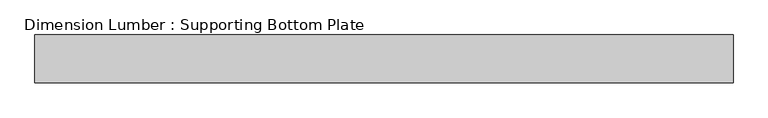
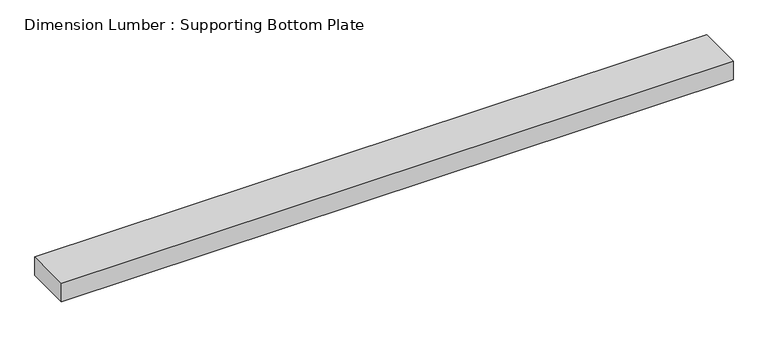
"""IFC4 building model written with IfcOpenShell, lengths in millimetres: beam geometry, Dimension Lumber : Supporting Bottom Plate."""

from ifc_helpers import new_model, si_unit, frame, origin, place, context, project, spatial, polyline, outline, extrude, source, transform, mapped, element, save


def dimension_lumber_supporting_bottom_plate_e800ad33(model_context):
    return source(origin(), model_context, "Body", "SweptSolid", [
        extrude(outline(polyline([(671.115625, 44.45), (671.115625, -44.45), (-626.665625, -44.45), (-626.665625, 44.45), (671.115625, 44.45)])), frame((0.0, 0.0, -19.05), z_axis=(0.0, 0.0, 1.0), x_axis=(1.0, 0.0, 0.0)), (0.0, 0.0, 1.0), 38.1),
    ])


if __name__ == "__main__":
    model = new_model("IFC4")
    model_context = context("Model", 3, world=origin())
    ifc_project = project(units=[si_unit("LENGTHUNIT", "METRE", prefix="MILLI")], contexts=[model_context])
    site = spatial("IfcSite", under=ifc_project)
    building = spatial("IfcBuilding", under=site)
    placement = place(None, origin())
    dimension_lumber_supporting_bottom_plate_shape = dimension_lumber_supporting_bottom_plate_e800ad33(model_context)
    element("IfcBeam", 1, ObjectType="Dimension Lumber : Supporting Bottom Plate", at=placement, inside=building, context=model_context, shape_type="MappedRepresentation", body=[
        mapped(dimension_lumber_supporting_bottom_plate_shape, transform((0.0, 0.0, 0.0), x_axis=(1.0, 0.0, 0.0), y_axis=(0.0, 1.0, 0.0), z_axis=(0.0, 0.0, 1.0))),
    ])
    save(model, "model.ifc")

# Revit data of these elements
# Type "Dimension Lumber : Supporting Bottom Plate"
#   Assembly Code = "B10"
#   A = 0.0364583 SF
#   Length [instance default] = 5' - 0"
#   b = 0' - 3 1/2"
#   d = 0' - 1 1/2"
#   Structural Material [instance default] = Softwood, Lumber
# Element 1 (IfcBeam, "Dimension Lumber : Supporting Bottom Plate")
#   Structural Material = Douglas Fir #2
#   Materials on its faces: "Douglas Fir #2"
# Materials
#   "Softwood, Lumber": class "Wood", colour RGB 223 192 134, transparency 0, Description = "Pinus Echinata", Cost = 0
#   "Douglas Fir #2": class "Wood", colour RGB 223 192 134, transparency 0, Description = "Pinus Echinata", Cost = 0
